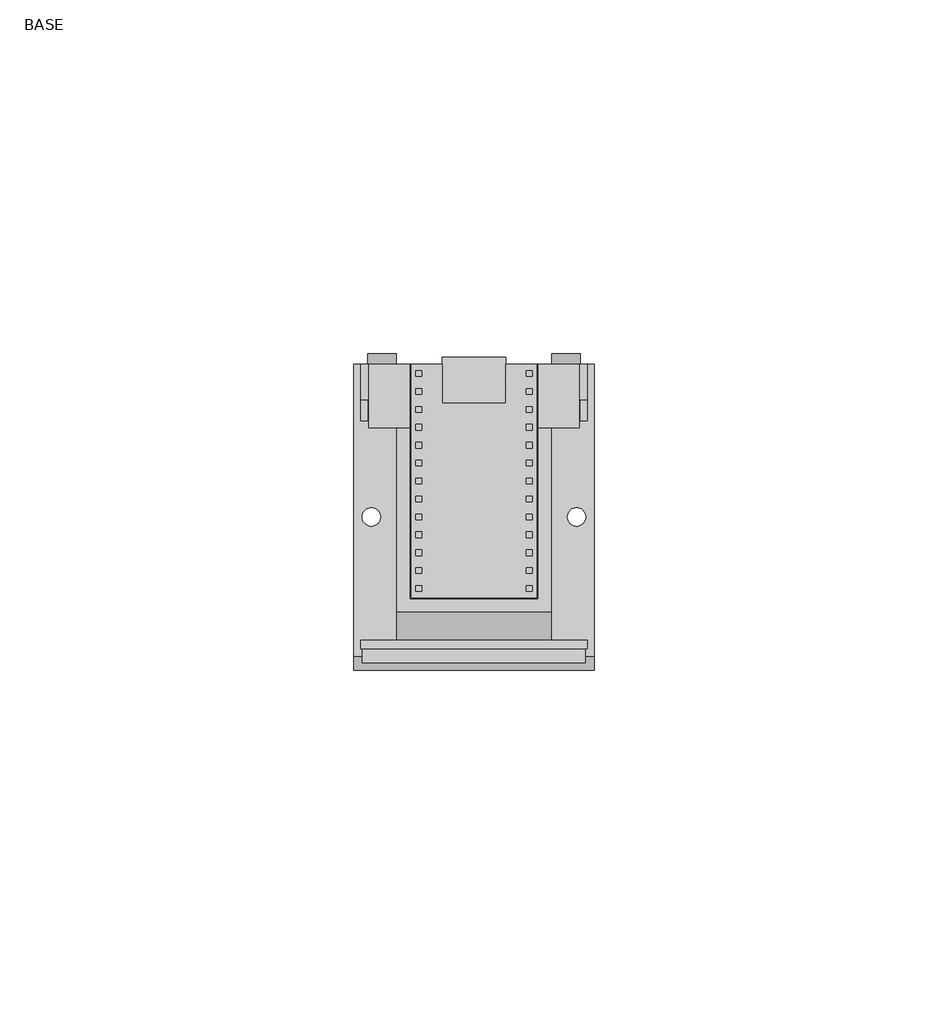
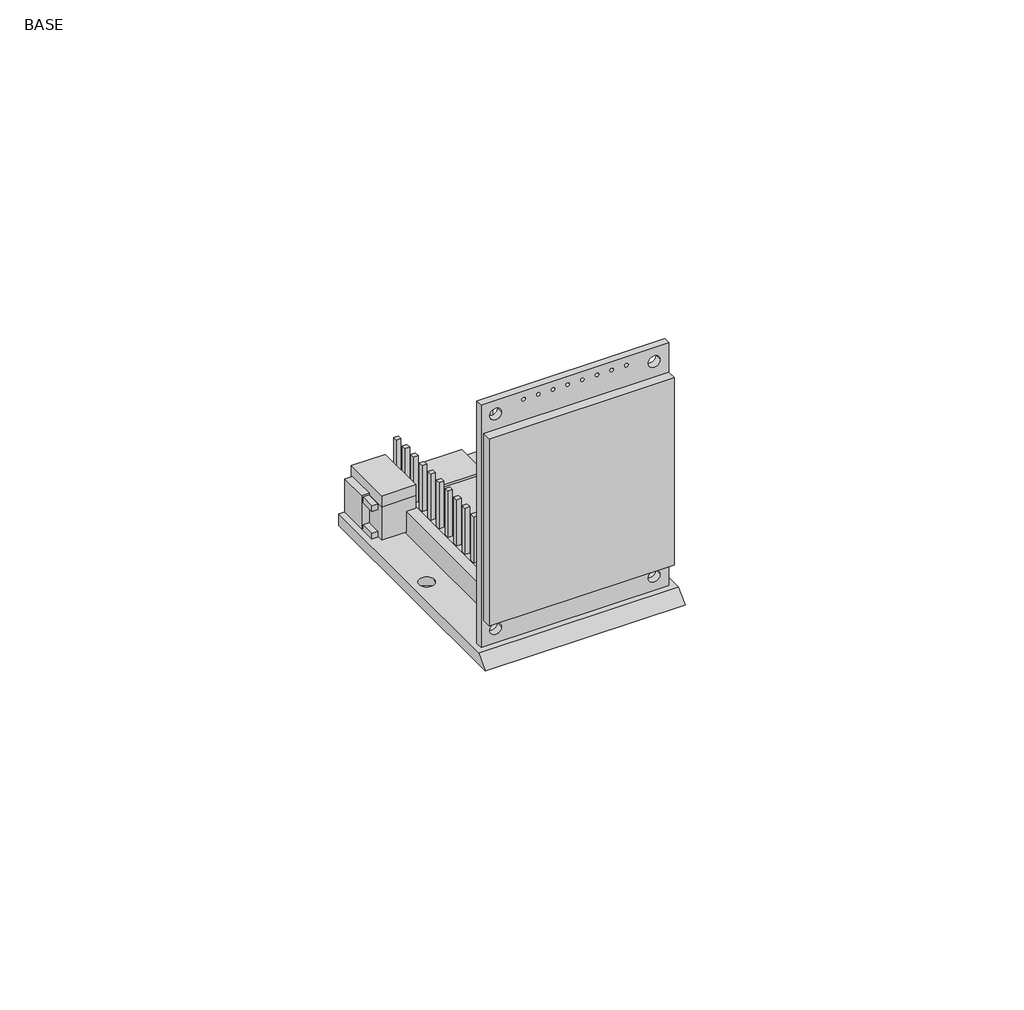
# One storey: 4 furniture elements, 1 proxy.
"""IFC4 building model written with IfcOpenShell, lengths in millimetres."""

import ifcopenshell
import ifcopenshell.guid

model = None  # the IFC model being written
_history = None  # IfcOwnerHistory: only IFC2X3 demands one
_inside = {}  # id of a spatial element -> (the spatial element, [elements in it])
_under = {}  # id of a project, library or spatial element -> (it, [spatial elements below it])
_declared = {}  # id of a project -> (the project, [libraries it declares])
_typed = {}  # id of a type object -> (the type object, [elements of that type])
_made_of = {}  # id of a material, layer set ... -> (it, [elements and type objects made of it])


def new_model(schema):
    """Start an empty IFC model of exactly this schema.

    Asked for "IFC4X3", IfcOpenShell would pick the latest addendum, in which some entities
    have other attributes; the version numbers below select the first issue.
    IFC2X3 requires an IfcOwnerHistory on every rooted entity: one is made here for all.
    """
    global model, _history
    if schema == "IFC4X3":
        model = ifcopenshell.file(schema_version=(4, 3, 0, 0))
    else:
        model = ifcopenshell.file(schema=schema)
    _inside.clear()
    _under.clear()
    _declared.clear()
    _typed.clear()
    _made_of.clear()
    _history = None
    if model.schema == "IFC2X3":
        org = make("IfcOrganization", Name="unknown")
        user = make(
            "IfcPersonAndOrganization",
            ThePerson=make("IfcPerson", FamilyName="unknown"),
            TheOrganization=org,
        )
        app = make(
            "IfcApplication",
            ApplicationDeveloper=org,
            Version="unknown",
            ApplicationFullName="unknown",
            ApplicationIdentifier="unknown",
        )
        _history = make(
            "IfcOwnerHistory",
            OwningUser=user,
            OwningApplication=app,
            ChangeAction="ADDED",
            CreationDate=0,
        )
    return model


def make(cls, **values):
    """One entity of the class cls with the attributes given. An attribute that is None is left unset."""
    return model.create_entity(
        cls, **{name: value for name, value in values.items() if value is not None}
    )


def rooted(cls, **values):
    """An entity with a GlobalId (a new one), such as an element, a storey or a relation."""
    return make(cls, GlobalId=ifcopenshell.guid.new(), OwnerHistory=_history, **values)


def si_unit(unit_type, name, prefix=None):
    """IfcSIUnit, for example si_unit("LENGTHUNIT", "METRE", prefix="MILLI")."""
    return make("IfcSIUnit", UnitType=unit_type, Prefix=prefix, Name=name)


def assignment(units):
    """IfcUnitAssignment: the units of a project."""
    return None if units is None else make("IfcUnitAssignment", Units=units)


def point(xyz):
    """IfcCartesianPoint."""
    return None if xyz is None else make("IfcCartesianPoint", Coordinates=xyz)


def direction(xyz):
    """IfcDirection."""
    return None if xyz is None else make("IfcDirection", DirectionRatios=xyz)


def frame(location, z_axis=None, x_axis=None):
    """IfcAxis2Placement3D, a coordinate frame: its origin and axes. An axis left out is left unset."""
    return make(
        "IfcAxis2Placement3D",
        Location=point(location),
        Axis=direction(z_axis),
        RefDirection=direction(x_axis),
    )


def frame_2d(location, x_axis=None):
    """IfcAxis2Placement2D, a coordinate frame in the plane: its origin and x axis."""
    return make(
        "IfcAxis2Placement2D", Location=point(location), RefDirection=direction(x_axis)
    )


def origin():
    """The frame at (0, 0, 0) with its axes left unset."""
    return frame((0.0, 0.0, 0.0))


def origin_with_axes():
    """The frame at (0, 0, 0) with the z axis (0, 0, 1) and the x axis (1, 0, 0) written out."""
    return frame((0.0, 0.0, 0.0), z_axis=(0.0, 0.0, 1.0), x_axis=(1.0, 0.0, 0.0))


def place(relative_to, where):
    """IfcLocalPlacement: puts the frame where relative to a parent placement (None: the world)."""
    return make(
        "IfcLocalPlacement", PlacementRelTo=relative_to, RelativePlacement=where
    )


def context(
    kind, dimensions, precision=None, world=None, true_north=None, identifier=None
):
    """IfcGeometricRepresentationContext, for example the 3D "Model" context."""
    return make(
        "IfcGeometricRepresentationContext",
        ContextIdentifier=identifier,
        ContextType=kind,
        CoordinateSpaceDimension=dimensions,
        Precision=precision,
        WorldCoordinateSystem=world,
        TrueNorth=true_north,
    )


def project(units=None, contexts=None):
    """IfcProject with its units and contexts."""
    return rooted(
        "IfcProject",
        Name="project",
        RepresentationContexts=contexts,
        UnitsInContext=assignment(units),
    )


def spatial(cls, under=None, at=None, **own):
    """A site, building, storey or space (cls), placed at a placement, below another one or the project."""
    s = rooted(cls, ObjectPlacement=at, **own)
    if under is not None:
        _under.setdefault(under.id(), (under, []))[1].append(s)
    return s


def polyline(points):
    """IfcPolyline through the points."""
    return make("IfcPolyline", Points=[point(p) for p in points])


def circle_curve(where, radius):
    """IfcCircle in the frame where."""
    return make("IfcCircle", Position=where, Radius=radius)


def trimmed(basis, trim1, trim2, sense, master):
    """IfcTrimmedCurve: the piece of a basis curve between two trims."""
    return make(
        "IfcTrimmedCurve",
        BasisCurve=basis,
        Trim1=trim1,
        Trim2=trim2,
        SenseAgreement=sense,
        MasterRepresentation=master,
    )


def segment(curve, same_sense, transition):
    """IfcCompositeCurveSegment."""
    return make(
        "IfcCompositeCurveSegment",
        Transition=transition,
        SameSense=same_sense,
        ParentCurve=curve,
    )


def composite_curve(segments, self_intersect=None):
    """IfcCompositeCurve: segments joined end to end."""
    return make("IfcCompositeCurve", Segments=segments, SelfIntersect=self_intersect)


def outline(outer, holes=None, kind="AREA"):
    """IfcArbitraryClosedProfileDef: a profile drawn as a closed curve; with holes, ...WithVoids."""
    if holes is None:
        return make("IfcArbitraryClosedProfileDef", ProfileType=kind, OuterCurve=outer)
    return make(
        "IfcArbitraryProfileDefWithVoids",
        ProfileType=kind,
        OuterCurve=outer,
        InnerCurves=holes,
    )


def extrude(swept, where, along, depth):
    """IfcExtrudedAreaSolid: the profile swept, set in the frame where, extruded along a direction by depth."""
    return make(
        "IfcExtrudedAreaSolid",
        SweptArea=swept,
        Position=where,
        ExtrudedDirection=direction(along),
        Depth=depth,
    )


def faces_of(points, faces, orient=None, outer=None):
    """IfcFace entities. A face is a list of loops; a loop is a list of indices into points, from 0.

    orient and outer hold one flag for each loop. By default every Orientation is true, the
    first loop of a face is its IfcFaceOuterBound and the others are IfcFaceBound.
    """
    made = []
    for i, loops in enumerate(faces):
        bounds = []
        for j, loop in enumerate(loops):
            is_outer = j == 0 if outer is None else outer[i][j]
            bounds.append(
                make(
                    "IfcFaceOuterBound" if is_outer else "IfcFaceBound",
                    Bound=make("IfcPolyLoop", Polygon=[points[k] for k in loop]),
                    Orientation=True if orient is None else orient[i][j],
                )
            )
        made.append(make("IfcFace", Bounds=bounds))
    return made


def faceted_brep(points, faces, orient=None, outer=None, voids=None):
    """IfcFacetedBrep: a solid bounded by flat faces; with voids (closed shells), ...WithVoids."""
    shared = [point(p) for p in points]
    hull = make("IfcClosedShell", CfsFaces=faces_of(shared, faces, orient, outer))
    if voids is None:
        return make("IfcFacetedBrep", Outer=hull)
    return make(
        "IfcFacetedBrepWithVoids",
        Outer=hull,
        Voids=[
            make(cls, CfsFaces=faces_of(shared, fs, o, b)) for cls, fs, o, b in voids
        ],
    )


def shape(context_of_items, identifier, shape_type, items):
    """IfcShapeRepresentation: the items that make up one representation, for example the "Body"."""
    return make(
        "IfcShapeRepresentation",
        ContextOfItems=context_of_items,
        RepresentationIdentifier=identifier,
        RepresentationType=shape_type,
        Items=items,
    )


def source(mapping_origin, context_of_items, identifier, shape_type, items):
    """IfcRepresentationMap: a shape defined once, which mapped items show again and again."""
    return make(
        "IfcRepresentationMap",
        MappingOrigin=mapping_origin,
        MappedRepresentation=shape(context_of_items, identifier, shape_type, items),
    )


def transform(
    local_origin,
    x_axis=None,
    y_axis=None,
    z_axis=None,
    scale=None,
    scale2=None,
    scale3=None,
    uniform=True,
):
    """IfcCartesianTransformationOperator3D, or its non-uniform kind. x_axis, y_axis, z_axis: its Axis1, 2, 3."""
    if uniform:
        return make(
            "IfcCartesianTransformationOperator3D",
            Axis1=direction(x_axis),
            Axis2=direction(y_axis),
            LocalOrigin=point(local_origin),
            Scale=scale,
            Axis3=direction(z_axis),
        )
    return make(
        "IfcCartesianTransformationOperator3DnonUniform",
        Axis1=direction(x_axis),
        Axis2=direction(y_axis),
        LocalOrigin=point(local_origin),
        Scale=scale,
        Axis3=direction(z_axis),
        Scale2=scale2,
        Scale3=scale3,
    )


def mapped(mapping_source, mapping_target):
    """IfcMappedItem: shows the shape of a source again, moved by a transform."""
    return make(
        "IfcMappedItem", MappingSource=mapping_source, MappingTarget=mapping_target
    )


def made_of(thing, what):
    """Note that an element or type object is made of a material, layer set ...; save() writes the relation."""
    if what is not None:
        _made_of.setdefault(what.id(), (what, []))[1].append(thing)
    return thing


def element(
    cls,
    number,
    at=None,
    inside=None,
    cuts=None,
    type_object=None,
    material=None,
    context=None,
    identifier="Body",
    shape_type=None,
    held_by="IfcProductDefinitionShape",
    body=None,
    shapes=None,
    **own,
):
    """One element of the class cls, such as IfcWall. Its Tag is "e" and its number.

    at: its placement. inside: the storey or other place that contains it. cuts: it is an
    opening in that element (IfcRelVoidsElement). A single representation is given by context,
    identifier, shape_type and body (its items); several are given by shapes. held_by: the class
    of the entity that holds the representations. save() writes the other relations.
    """
    e = rooted(cls, Tag="e%d" % number, ObjectPlacement=at, **own)
    if body is not None:
        shapes = [shape(context, identifier, shape_type, body)]
    if shapes is not None:
        e.Representation = make(held_by, Representations=shapes)
    if inside is not None:
        _inside.setdefault(inside.id(), (inside, []))[1].append(e)
    if cuts is not None:
        rooted(
            "IfcRelVoidsElement", RelatingBuildingElement=cuts, RelatedOpeningElement=e
        )
    if type_object is not None:
        _typed.setdefault(type_object.id(), (type_object, []))[1].append(e)
    return made_of(e, material)


def aggregate(whole, parts):
    """IfcRelAggregates: a whole, such as a stair, and the parts it consists of."""
    return rooted("IfcRelAggregates", RelatingObject=whole, RelatedObjects=parts)


def save(model, path):
    """Write the relations noted so far, then the file.

    IfcRelAggregates (storeys below a building ...), IfcRelContainedInSpatialStructure (elements
    in a storey), IfcRelDefinesByType, IfcRelAssociatesMaterial and IfcRelDeclares: one each for
    every whole, place, type object, material and project.
    """
    for whole, parts in _under.values():
        aggregate(whole, parts)
    for where, things in _inside.values():
        rooted(
            "IfcRelContainedInSpatialStructure",
            RelatedElements=things,
            RelatingStructure=where,
        )
    for kind, things in _typed.values():
        rooted("IfcRelDefinesByType", RelatedObjects=things, RelatingType=kind)
    for what, things in _made_of.values():
        rooted("IfcRelAssociatesMaterial", RelatedObjects=things, RelatingMaterial=what)
    for by, libraries in _declared.values():
        rooted("IfcRelDeclares", RelatingContext=by, RelatedDefinitions=libraries)
    model.write(path)


def plane_surface(at):
    """IfcPlane: the flat surface through the origin of the frame at, square to its z axis."""
    return make("IfcPlane", Position=at)


def revolved_surface(curve, axis_point, axis_direction):
    """IfcSurfaceOfRevolution: the curve turned about the line through axis_point along axis_direction."""
    return make(
        "IfcSurfaceOfRevolution",
        SweptCurve=make("IfcArbitraryOpenProfileDef", ProfileType="CURVE", Curve=curve),
        AxisPosition=make("IfcAxis1Placement", Location=point(axis_point), Axis=direction(axis_direction)),
    )


def advanced_brep(points, edges, surfaces, faces):
    """IfcAdvancedBrep: a solid bounded by faces that lie on surfaces and meet in shared edges.

    An edge is (start, end): straight between two places in points (the first is 0);
    or (start, end, curve); or (start, end, curve, False) where it runs against its curve.
    A face is (place in surfaces, loops), or (place, loops, False) where it looks against
    its surface's normal. A loop lists edges by number (the first is 1), with a minus sign
    where the edge is run from its end to its start. The first loop is the outer one.
    """
    corners = [point(p) for p in points]
    vertices = [make("IfcVertexPoint", VertexGeometry=c) for c in corners]
    made = []
    for start, end, *more in edges:
        made.append(
            make(
                "IfcEdgeCurve",
                EdgeStart=vertices[start],
                EdgeEnd=vertices[end],
                EdgeGeometry=more[0] if more else make("IfcPolyline", Points=[corners[start], corners[end]]),
                SameSense=more[1] if len(more) > 1 else True,
            )
        )
    hull = []
    for where, loops, *sense in faces:
        bounds = []
        for j, loop in enumerate(loops):
            ring = [make("IfcOrientedEdge", EdgeElement=made[abs(k) - 1], Orientation=k > 0) for k in loop]
            bounds.append(
                make(
                    "IfcFaceOuterBound" if j == 0 else "IfcFaceBound",
                    Bound=make("IfcEdgeLoop", EdgeList=ring),
                    Orientation=True,
                )
            )
        hull.append(make("IfcAdvancedFace", Bounds=bounds, FaceSurface=surfaces[where], SameSense=sense[0] if sense else True))
    return make("IfcAdvancedBrep", Outer=make("IfcClosedShell", CfsFaces=hull))


def case_case_fa127987(model_context):
    return source(origin(), model_context, "Body", "SolidModel", [
        extrude(outline(polyline([(1442.9350176, 13234.6739696), (1442.9350176, 13225.7186096), (1437.1350176, 13225.7186096), (1437.1350176, 13234.6739696), (1442.9350176, 13234.6739696)])), frame((0.0, 0.0, 8.0), z_axis=(0.0, 0.0, 1.0), x_axis=(1.0, 0.0, 0.0)), (0.0, 0.0, 1.0), 2.0),
        extrude(outline(polyline([(1461.1150176, 13234.6739696), (1466.9150176, 13234.6739696), (1466.9150176, 13225.7186096), (1461.1150176, 13225.7186096), (1461.1150176, 13234.6739696)])), frame((0.0, 0.0, 8.0), z_axis=(0.0, 0.0, 1.0), x_axis=(1.0, 0.0, 0.0)), (0.0, 0.0, 1.0), 2.0),
        extrude(outline(polyline([(1442.9350176, 13230.2186096), (1442.9350176, 13225.7186096), (1437.1350176, 13225.7186096), (1437.1350176, 13230.2186096), (1442.9350176, 13230.2186096)])), frame((0.0, 0.0, 2.0), z_axis=(0.0, 0.0, 1.0), x_axis=(1.0, 0.0, 0.0)), (0.0, 0.0, 1.0), 6.0),
        extrude(outline(polyline([(1461.1150176, 13230.2186096), (1466.9150176, 13230.2186096), (1466.9150176, 13225.7186096), (1461.1150176, 13225.7186096), (1461.1150176, 13230.2186096)])), frame((0.0, 0.0, 2.0), z_axis=(0.0, 0.0, 1.0), x_axis=(1.0, 0.0, 0.0)), (0.0, 0.0, 1.0), 6.0),
        advanced_brep(
        [(1469.0250176, 13193.4256546, 2.0), (1469.0250176, 13234.6739696, 2.0), (1435.0250176, 13234.6739696, 2.0), (1435.0250176, 13193.4256546, 2.0), (1441.1350176, 13195.6739696, 2.0), (1441.1350176, 13225.7186096, 2.0), (1442.9350176, 13225.7186096, 2.0), (1442.9350176, 13201.4739696, 2.0), (1461.1150176, 13201.4739696, 2.0), (1461.1150176, 13225.7186096, 2.0), (1462.9150176, 13225.7186096, 2.0), (1462.9150176, 13195.6739696, 2.0), (1467.8250176, 13213.1041412, 2.0), (1465.2250176, 13213.1041412, 2.0), (1438.8250176, 13213.1041412, 2.0), (1436.2250176, 13213.1041412, 2.0), (1435.0250176, 13234.6739696, 0.0), (1469.0250176, 13234.6739696, 0.0), (1469.0250176, 13191.4256546, 0.0), (1435.0250176, 13191.4256546, 0.0), (1464.5250176, 13213.1041412, 0.0), (1468.5250176, 13213.1041412, 0.0), (1435.5250176, 13213.1041412, 0.0), (1439.5250176, 13213.1041412, 0.0), (1441.1350176, 13225.7186096, 6.0), (1441.1350176, 13199.6739696, 6.0), (1462.9150176, 13199.6739696, 6.0), (1462.9150176, 13225.7186096, 6.0), (1461.1150176, 13225.7186096, 6.0), (1461.1150176, 13201.4739696, 6.0), (1442.9350176, 13201.4739696, 6.0), (1442.9350176, 13225.7186096, 6.0)],
        [
            (0, 1),
            (1, 2),
            (2, 3),
            (3, 0),
            (4, 5),
            (5, 6),
            (6, 7),
            (7, 8),
            (8, 9),
            (9, 10),
            (10, 11),
            (11, 4),
            (12, 13, circle_curve(frame((1466.5250176, 13213.1041412, 2.0), z_axis=(0.0, 0.0, -1.0), x_axis=(-1.0, 0.0, 0.0)), 1.3)),
            (13, 12, circle_curve(frame((1466.5250176, 13213.1041412, 2.0), z_axis=(0.0, 0.0, -1.0), x_axis=(1.0, 0.0, 0.0)), 1.3)),
            (14, 15, circle_curve(frame((1437.5250176, 13213.1041412, 2.0), z_axis=(0.0, 0.0, -1.0), x_axis=(-1.0, 0.0, 0.0)), 1.3)),
            (15, 14, circle_curve(frame((1437.5250176, 13213.1041412, 2.0), z_axis=(0.0, 0.0, -1.0), x_axis=(1.0, 0.0, 0.0)), 1.3)),
            (16, 17),
            (17, 18),
            (18, 19),
            (19, 16),
            (20, 21, circle_curve(frame((1466.5250176, 13213.1041412, 0.0), z_axis=(0.0, 0.0, 1.0), x_axis=(-1.0, 0.0, 0.0)), 2.0)),
            (21, 20, circle_curve(frame((1466.5250176, 13213.1041412, 0.0), z_axis=(0.0, 0.0, 1.0), x_axis=(1.0, 0.0, 0.0)), 2.0)),
            (22, 23, circle_curve(frame((1437.5250176, 13213.1041412, 0.0), z_axis=(0.0, 0.0, 1.0), x_axis=(-1.0, 0.0, 0.0)), 2.0)),
            (23, 22, circle_curve(frame((1437.5250176, 13213.1041412, 0.0), z_axis=(0.0, 0.0, 1.0), x_axis=(1.0, 0.0, 0.0)), 2.0)),
            (0, 18),
            (17, 1),
            (16, 2),
            (19, 3),
            (24, 25),
            (25, 26),
            (26, 27),
            (27, 28),
            (28, 29),
            (29, 30),
            (30, 31),
            (31, 24),
            (24, 5),
            (4, 25),
            (26, 11),
            (10, 27),
            (9, 28),
            (8, 29),
            (7, 30),
            (6, 31),
            (20, 13),
            (12, 21),
            (22, 15),
            (14, 23),
        ],
        [
            plane_surface(frame((1467.7850176, 13193.4256546, 2.0), z_axis=(0.0, 0.0, 1.0), x_axis=(1.0, 0.0, 0.0))),
            plane_surface(frame((1467.7850176, 13193.4256546, 0.0), z_axis=(0.0, 0.0, -1.0), x_axis=(-1.0, 0.0, 0.0))),
            plane_surface(frame((1469.0250176, 13193.4256546, 2.0), z_axis=(1.0, 0.0, 0.0), x_axis=(0.0, 0.0, -1.0))),
            plane_surface(frame((1469.0250176, 13234.6739696, 2.0), z_axis=(0.0, 1.0, 0.0), x_axis=(0.0, 0.0, -1.0))),
            plane_surface(frame((1435.0250176, 13234.6739696, 2.0), z_axis=(-1.0, 0.0, 0.0), x_axis=(0.0, 0.0, -1.0))),
            plane_surface(frame((1441.1350176, 13234.6739696, 6.0), z_axis=(0.0, 0.0, 1.0), x_axis=(0.0, -1.0, 0.0))),
            plane_surface(frame((1441.1350176, 13225.7186096, 6.0), z_axis=(-1.0, 0.0, 0.0), x_axis=(0.0, 0.0, -1.0))),
            plane_surface(frame((1462.9150176, 13199.6739696, 6.0), z_axis=(1.0, 0.0, 0.0), x_axis=(0.0, 0.0, -1.0))),
            plane_surface(frame((1462.9150176, 13225.7186096, 6.0), z_axis=(0.0, 1.0, 0.0), x_axis=(0.0, 0.0, -1.0))),
            plane_surface(frame((1461.1150176, 13225.7186096, 6.0), z_axis=(-1.0, 0.0, 0.0), x_axis=(0.0, 0.0, -1.0))),
            plane_surface(frame((1461.1150176, 13201.4739696, 6.0), z_axis=(0.0, 1.0, 0.0), x_axis=(0.0, 0.0, -1.0))),
            plane_surface(frame((1442.9350176, 13201.4739696, 6.0), z_axis=(1.0, 0.0, 0.0), x_axis=(0.0, 0.0, -1.0))),
            plane_surface(frame((1442.9350176, 13225.7186096, 6.0), z_axis=(0.0, 1.0, 0.0), x_axis=(0.0, 0.0, -1.0))),
            plane_surface(frame((1441.1350176, 13195.6739696, 2.0), z_axis=(0.0, -0.7071067811865885, 0.7071067811865066), x_axis=(1.0, 0.0, 0.0))),
            revolved_surface(polyline([(1464.5250176, 13213.1041412, 0.0), (1465.2250176017499, 13213.1041412, 2.0)]), (1466.5250176, 13213.1041412, 5.7142857), (0.0, 0.0, -1.0)),
            revolved_surface(polyline([(1435.5250176, 13213.1041412, 0.0), (1436.2250176017499, 13213.1041412, 2.0)]), (1437.5250176, 13213.1041412, 5.7142857), (0.0, 0.0, -1.0)),
            plane_surface(frame((1435.0250176, 13191.4256546, 0.0), z_axis=(0.0, -0.707106781186628, 0.7071067811864672), x_axis=(1.0, 0.0, 0.0))),
        ],
        [
            (0, [[1, 2, 3, 4], [5, 6, 7, 8, 9, 10, 11, 12], [13, 14], [15, 16]]),
            (1, [[17, 18, 19, 20], [21, 22], [23, 24]]),
            (2, [[-1, 25, -18, 26]]),
            (3, [[-2, -26, -17, 27]]),
            (4, [[-3, -27, -20, 28]]),
            (5, [[29, 30, 31, 32, 33, 34, 35, 36]]),
            (6, [[-29, 37, -5, 38]]),
            (7, [[-31, 39, -11, 40]]),
            (8, [[-32, -40, -10, 41]]),
            (9, [[-33, -41, -9, 42]]),
            (10, [[-34, -42, -8, 43]]),
            (11, [[-35, -43, -7, 44]]),
            (12, [[-36, -44, -6, -37]]),
            (13, [[-38, -12, -39, -30]]),
            (14, [[45, -13, 46, -21]]),
            (14, [[-45, -22, -46, -14]]),
            (15, [[47, -15, 48, -23]]),
            (15, [[-47, -24, -48, -16]]),
            (16, [[-28, -19, -25, -4]]),
        ],
    ),
    ])


def furniture_1_54tft_screen_1_54tft_screen_d9e98271(model_context):
    return source(origin(), model_context, "Body", "SweptSolid", [
        extrude(outline(polyline([(43.7, 16.0), (43.7, -16.0), (0.0, -16.0), (0.0, 16.0), (43.7, 16.0)]), holes=[composite_curve([segment(trimmed(circle_curve(frame_2d((2.5, 13.5)), 1.0), [point((2.5, 14.5))], [point((2.5, 12.5))], True, "CARTESIAN"), True, "CONTINUOUS"), segment(trimmed(circle_curve(frame_2d((2.5, 13.5)), 1.0), [point((2.5, 12.5))], [point((2.5, 14.5))], True, "CARTESIAN"), True, "CONTINUOUS")], self_intersect=False), composite_curve([segment(trimmed(circle_curve(frame_2d((41.2, 13.5)), 1.0), [point((41.2, 14.5))], [point((41.2, 12.5))], True, "CARTESIAN"), True, "CONTINUOUS"), segment(trimmed(circle_curve(frame_2d((41.2, 13.5)), 1.0), [point((41.2, 12.5))], [point((41.2, 14.5))], True, "CARTESIAN"), True, "CONTINUOUS")], self_intersect=False), composite_curve([segment(trimmed(circle_curve(frame_2d((42.2, -1.25)), 0.3), [point((42.2, -0.95))], [point((42.2, -1.55))], True, "CARTESIAN"), True, "CONTINUOUS"), segment(trimmed(circle_curve(frame_2d((42.2, -1.25)), 0.3), [point((42.2, -1.55))], [point((42.2, -0.95))], True, "CARTESIAN"), True, "CONTINUOUS")], self_intersect=False), composite_curve([segment(trimmed(circle_curve(frame_2d((42.2, 1.25)), 0.3), [point((42.2, 1.55))], [point((42.2, 0.95))], True, "CARTESIAN"), True, "CONTINUOUS"), segment(trimmed(circle_curve(frame_2d((42.2, 1.25)), 0.3), [point((42.2, 0.95))], [point((42.2, 1.55))], True, "CARTESIAN"), True, "CONTINUOUS")], self_intersect=False), composite_curve([segment(trimmed(circle_curve(frame_2d((42.2, 3.75)), 0.3), [point((42.2, 4.05))], [point((42.2, 3.45))], True, "CARTESIAN"), True, "CONTINUOUS"), segment(trimmed(circle_curve(frame_2d((42.2, 3.75)), 0.3), [point((42.2, 3.45))], [point((42.2, 4.05))], True, "CARTESIAN"), True, "CONTINUOUS")], self_intersect=False), composite_curve([segment(trimmed(circle_curve(frame_2d((42.2, 6.25)), 0.3), [point((42.2, 6.55))], [point((42.2, 5.95))], True, "CARTESIAN"), True, "CONTINUOUS"), segment(trimmed(circle_curve(frame_2d((42.2, 6.25)), 0.3), [point((42.2, 5.95))], [point((42.2, 6.55))], True, "CARTESIAN"), True, "CONTINUOUS")], self_intersect=False), composite_curve([segment(trimmed(circle_curve(frame_2d((42.2, 8.75)), 0.3), [point((42.2, 9.05))], [point((42.2, 8.45))], True, "CARTESIAN"), True, "CONTINUOUS"), segment(trimmed(circle_curve(frame_2d((42.2, 8.75)), 0.3), [point((42.2, 8.45))], [point((42.2, 9.05))], True, "CARTESIAN"), True, "CONTINUOUS")], self_intersect=False), composite_curve([segment(trimmed(circle_curve(frame_2d((42.2, -3.75)), 0.3), [point((42.2, -3.45))], [point((42.2, -4.05))], True, "CARTESIAN"), True, "CONTINUOUS"), segment(trimmed(circle_curve(frame_2d((42.2, -3.75)), 0.3), [point((42.2, -4.05))], [point((42.2, -3.45))], True, "CARTESIAN"), True, "CONTINUOUS")], self_intersect=False), composite_curve([segment(trimmed(circle_curve(frame_2d((42.2, -6.25)), 0.3), [point((42.2, -5.95))], [point((42.2, -6.55))], True, "CARTESIAN"), True, "CONTINUOUS"), segment(trimmed(circle_curve(frame_2d((42.2, -6.25)), 0.3), [point((42.2, -6.55))], [point((42.2, -5.95))], True, "CARTESIAN"), True, "CONTINUOUS")], self_intersect=False), composite_curve([segment(trimmed(circle_curve(frame_2d((42.2, -8.75)), 0.3), [point((42.2, -8.45))], [point((42.2, -9.05))], True, "CARTESIAN"), True, "CONTINUOUS"), segment(trimmed(circle_curve(frame_2d((42.2, -8.75)), 0.3), [point((42.2, -9.05))], [point((42.2, -8.45))], True, "CARTESIAN"), True, "CONTINUOUS")], self_intersect=False), composite_curve([segment(trimmed(circle_curve(frame_2d((41.2, -13.5)), 1.0), [point((41.2, -14.5))], [point((41.2, -12.5))], True, "CARTESIAN"), True, "CONTINUOUS"), segment(trimmed(circle_curve(frame_2d((41.2, -13.5)), 1.0), [point((41.2, -12.5))], [point((41.2, -14.5))], True, "CARTESIAN"), True, "CONTINUOUS")], self_intersect=False), composite_curve([segment(trimmed(circle_curve(frame_2d((2.5, -13.5)), 1.0), [point((2.5, -14.5))], [point((2.5, -12.5))], True, "CARTESIAN"), True, "CONTINUOUS"), segment(trimmed(circle_curve(frame_2d((2.5, -13.5)), 1.0), [point((2.5, -12.5))], [point((2.5, -14.5))], True, "CARTESIAN"), True, "CONTINUOUS")], self_intersect=False)]), frame((0.0, -1.2, 0.0), z_axis=(0.0, 1.0, 0.0), x_axis=(0.0, 0.0, 1.0)), (0.0, 0.0, 1.0), 1.2),
        extrude(outline(polyline([(15.76, -1.3), (15.76, -3.2), (-15.76, -3.2), (-15.76, -1.3), (15.76, -1.3)])), frame((0.0, 0.0, 5.0), z_axis=(0.0, 0.0, 1.0), x_axis=(1.0, 0.0, 0.0)), (0.0, 0.0, 1.0), 33.7),
        extrude(outline(polyline([(13.86, -2.3592442), (13.86, -3.2), (-13.86, -3.2), (-13.86, -2.3592442), (13.86, -2.3592442)])), frame((0.0, 0.0, 9.5994076), z_axis=(0.0, 0.0, 1.0), x_axis=(1.0, 0.0, 0.0)), (0.0, 0.0, 1.0), 27.7),
    ])


def pro_micro_nrf52840_pro_micro_nrf52840_bcfd0b97(model_context):
    return source(origin(), model_context, "Body", "Brep", [
        faceted_brep([(-14.8, 8.2144911, 11.3), (-15.6, 8.2144911, 11.3), (-15.6, 7.4144911, 11.3), (-14.8, 7.4144911, 11.3), (15.6, 8.2144911, 11.3), (14.8, 8.2144911, 11.3), (14.8, 7.4144911, 11.3), (15.6, 7.4144911, 11.3), (13.0666667, 8.2144911, 11.3), (12.2666667, 8.2144911, 11.3), (12.2666667, 7.4144911, 11.3), (13.0666667, 7.4144911, 11.3), (10.5333333, 8.2144911, 11.3), (9.7333333, 8.2144911, 11.3), (9.7333333, 7.4144911, 11.3), (10.5333333, 7.4144911, 11.3), (8.0, 8.2144911, 11.3), (7.2, 8.2144911, 11.3), (7.2, 7.4144911, 11.3), (8.0, 7.4144911, 11.3), (5.4666667, 8.2144911, 11.3), (4.6666667, 8.2144911, 11.3), (4.6666667, 7.4144911, 11.3), (5.4666667, 7.4144911, 11.3), (2.9333333, 8.2144911, 11.3), (2.1333333, 8.2144911, 11.3), (2.1333333, 7.4144911, 11.3), (2.9333333, 7.4144911, 11.3), (0.4, 8.2144911, 11.3), (-0.4, 8.2144911, 11.3), (-0.4, 7.4144911, 11.3), (0.4, 7.4144911, 11.3), (-2.1333333, 8.2144911, 11.3), (-2.9333333, 8.2144911, 11.3), (-2.9333333, 7.4144911, 11.3), (-2.1333333, 7.4144911, 11.3), (-4.6666667, 8.2144911, 11.3), (-5.4666667, 8.2144911, 11.3), (-5.4666667, 7.4144911, 11.3), (-4.6666667, 7.4144911, 11.3), (-7.2, 8.2144911, 11.3), (-8.0, 8.2144911, 11.3), (-8.0, 7.4144911, 11.3), (-7.2, 7.4144911, 11.3), (-9.7333333, 8.2144911, 11.3), (-10.5333333, 8.2144911, 11.3), (-10.5333333, 7.4144911, 11.3), (-9.7333333, 7.4144911, 11.3), (-12.2666667, 8.2144911, 11.3), (-13.0666667, 8.2144911, 11.3), (-13.0666667, 7.4144911, 11.3), (-12.2666667, 7.4144911, 11.3), (-14.8, 8.2144911, 0.0), (-14.8, 7.4144911, 0.0), (-15.6, 7.4144911, 0.0), (-15.6, 8.2144911, 0.0), (15.6, 8.2144911, 0.0), (15.6, 7.4144911, 0.0), (14.8, 7.4144911, 0.0), (14.8, 8.2144911, 0.0), (13.0666667, 8.2144911, 0.0), (13.0666667, 7.4144911, 0.0), (12.2666667, 7.4144911, 0.0), (12.2666667, 8.2144911, 0.0), (10.5333333, 8.2144911, 0.0), (10.5333333, 7.4144911, 0.0), (9.7333333, 7.4144911, 0.0), (9.7333333, 8.2144911, 0.0), (8.0, 8.2144911, 0.0), (8.0, 7.4144911, 0.0), (7.2, 7.4144911, 0.0), (7.2, 8.2144911, 0.0), (5.4666667, 8.2144911, 0.0), (5.4666667, 7.4144911, 0.0), (4.6666667, 7.4144911, 0.0), (4.6666667, 8.2144911, 0.0), (2.9333333, 8.2144911, 0.0), (2.9333333, 7.4144911, 0.0), (2.1333333, 7.4144911, 0.0), (2.1333333, 8.2144911, 0.0), (0.4, 8.2144911, 0.0), (0.4, 7.4144911, 0.0), (-0.4, 7.4144911, 0.0), (-0.4, 8.2144911, 0.0), (-2.1333333, 8.2144911, 0.0), (-2.1333333, 7.4144911, 0.0), (-2.9333333, 7.4144911, 0.0), (-2.9333333, 8.2144911, 0.0), (-4.6666667, 8.2144911, 0.0), (-4.6666667, 7.4144911, 0.0), (-5.4666667, 7.4144911, 0.0), (-5.4666667, 8.2144911, 0.0), (-7.2, 8.2144911, 0.0), (-7.2, 7.4144911, 0.0), (-8.0, 7.4144911, 0.0), (-8.0, 8.2144911, 0.0), (-9.7333333, 8.2144911, 0.0), (-9.7333333, 7.4144911, 0.0), (-10.5333333, 7.4144911, 0.0), (-10.5333333, 8.2144911, 0.0), (-12.2666667, 8.2144911, 0.0), (-12.2666667, 7.4144911, 0.0), (-13.0666667, 7.4144911, 0.0), (-13.0666667, 8.2144911, 0.0), (-14.8, 8.2144911, 3.0), (-15.6, 8.2144911, 3.0), (-15.6, 8.2144911, 1.0), (-14.8, 8.2144911, 1.0), (-15.6, 7.4144911, 3.0), (-15.6, 7.4144911, 1.0), (-14.8, 7.4144911, 3.0), (-14.8, 7.4144911, 1.0), (15.6, 8.2144911, 3.0), (14.8, 8.2144911, 3.0), (14.8, 8.2144911, 1.0), (15.6, 8.2144911, 1.0), (14.8, 7.4144911, 3.0), (14.8, 7.4144911, 1.0), (15.6, 7.4144911, 3.0), (15.6, 7.4144911, 1.0), (13.0666667, 8.2144911, 3.0), (12.2666667, 8.2144911, 3.0), (12.2666667, 8.2144911, 1.0), (13.0666667, 8.2144911, 1.0), (12.2666667, 7.4144911, 3.0), (12.2666667, 7.4144911, 1.0), (13.0666667, 7.4144911, 3.0), (13.0666667, 7.4144911, 1.0), (10.5333333, 8.2144911, 3.0), (9.7333333, 8.2144911, 3.0), (9.7333333, 8.2144911, 1.0), (10.5333333, 8.2144911, 1.0), (9.7333333, 7.4144911, 3.0), (9.7333333, 7.4144911, 1.0), (10.5333333, 7.4144911, 3.0), (10.5333333, 7.4144911, 1.0), (8.0, 8.2144911, 3.0), (7.2, 8.2144911, 3.0), (7.2, 8.2144911, 1.0), (8.0, 8.2144911, 1.0), (7.2, 7.4144911, 3.0), (7.2, 7.4144911, 1.0), (8.0, 7.4144911, 3.0), (8.0, 7.4144911, 1.0), (5.4666667, 8.2144911, 3.0), (4.6666667, 8.2144911, 3.0), (4.6666667, 8.2144911, 1.0), (5.4666667, 8.2144911, 1.0), (4.6666667, 7.4144911, 3.0), (4.6666667, 7.4144911, 1.0), (5.4666667, 7.4144911, 3.0), (5.4666667, 7.4144911, 1.0), (2.9333333, 8.2144911, 3.0), (2.1333333, 8.2144911, 3.0), (2.1333333, 8.2144911, 1.0), (2.9333333, 8.2144911, 1.0), (2.1333333, 7.4144911, 3.0), (2.1333333, 7.4144911, 1.0), (2.9333333, 7.4144911, 3.0), (2.9333333, 7.4144911, 1.0), (0.4, 8.2144911, 3.0), (-0.4, 8.2144911, 3.0), (-0.4, 8.2144911, 1.0), (0.4, 8.2144911, 1.0), (-0.4, 7.4144911, 3.0), (-0.4, 7.4144911, 1.0), (0.4, 7.4144911, 3.0), (0.4, 7.4144911, 1.0), (-2.1333333, 8.2144911, 3.0), (-2.9333333, 8.2144911, 3.0), (-2.9333333, 8.2144911, 1.0), (-2.1333333, 8.2144911, 1.0), (-2.9333333, 7.4144911, 3.0), (-2.9333333, 7.4144911, 1.0), (-2.1333333, 7.4144911, 3.0), (-2.1333333, 7.4144911, 1.0), (-4.6666667, 8.2144911, 3.0), (-5.4666667, 8.2144911, 3.0), (-5.4666667, 8.2144911, 1.0), (-4.6666667, 8.2144911, 1.0), (-5.4666667, 7.4144911, 3.0), (-5.4666667, 7.4144911, 1.0), (-4.6666667, 7.4144911, 3.0), (-4.6666667, 7.4144911, 1.0), (-7.2, 8.2144911, 3.0), (-8.0, 8.2144911, 3.0), (-8.0, 8.2144911, 1.0), (-7.2, 8.2144911, 1.0), (-8.0, 7.4144911, 3.0), (-8.0, 7.4144911, 1.0), (-7.2, 7.4144911, 3.0), (-7.2, 7.4144911, 1.0), (-9.7333333, 8.2144911, 3.0), (-10.5333333, 8.2144911, 3.0), (-10.5333333, 8.2144911, 1.0), (-9.7333333, 8.2144911, 1.0), (-10.5333333, 7.4144911, 3.0), (-10.5333333, 7.4144911, 1.0), (-9.7333333, 7.4144911, 3.0), (-9.7333333, 7.4144911, 1.0), (-12.2666667, 8.2144911, 3.0), (-13.0666667, 8.2144911, 3.0), (-13.0666667, 8.2144911, 1.0), (-12.2666667, 8.2144911, 1.0), (-13.0666667, 7.4144911, 3.0), (-13.0666667, 7.4144911, 1.0), (-12.2666667, 7.4144911, 3.0), (-12.2666667, 7.4144911, 1.0), (16.5, 8.89, 3.0), (-16.5, 8.89, 3.0), (-16.5, -8.89, 3.0), (16.5, -8.89, 3.0), (16.5, -4.5, 3.0), (11.0, -4.5, 3.0), (11.0, 4.5, 3.0), (16.5, 4.5, 3.0), (-14.8, -8.2144911, 3.0), (-15.6, -8.2144911, 3.0), (-15.6, -7.4144911, 3.0), (-14.8, -7.4144911, 3.0), (15.6, -8.2144911, 3.0), (14.8, -8.2144911, 3.0), (14.8, -7.4144911, 3.0), (15.6, -7.4144911, 3.0), (13.0666667, -8.2144911, 3.0), (12.2666667, -8.2144911, 3.0), (12.2666667, -7.4144911, 3.0), (13.0666667, -7.4144911, 3.0), (10.5333333, -8.2144911, 3.0), (9.7333333, -8.2144911, 3.0), (9.7333333, -7.4144911, 3.0), (10.5333333, -7.4144911, 3.0), (8.0, -8.2144911, 3.0), (7.2, -8.2144911, 3.0), (7.2, -7.4144911, 3.0), (8.0, -7.4144911, 3.0), (5.4666667, -8.2144911, 3.0), (4.6666667, -8.2144911, 3.0), (4.6666667, -7.4144911, 3.0), (5.4666667, -7.4144911, 3.0), (2.9333333, -8.2144911, 3.0), (2.1333333, -8.2144911, 3.0), (2.1333333, -7.4144911, 3.0), (2.9333333, -7.4144911, 3.0), (0.4, -8.2144911, 3.0), (-0.4, -8.2144911, 3.0), (-0.4, -7.4144911, 3.0), (0.4, -7.4144911, 3.0), (-2.1333333, -8.2144911, 3.0), (-2.9333333, -8.2144911, 3.0), (-2.9333333, -7.4144911, 3.0), (-2.1333333, -7.4144911, 3.0), (-4.6666667, -8.2144911, 3.0), (-5.4666667, -8.2144911, 3.0), (-5.4666667, -7.4144911, 3.0), (-4.6666667, -7.4144911, 3.0), (-7.2, -8.2144911, 3.0), (-8.0, -8.2144911, 3.0), (-8.0, -7.4144911, 3.0), (-7.2, -7.4144911, 3.0), (-9.7333333, -8.2144911, 3.0), (-10.5333333, -8.2144911, 3.0), (-10.5333333, -7.4144911, 3.0), (-9.7333333, -7.4144911, 3.0), (-12.2666667, -8.2144911, 3.0), (-13.0666667, -8.2144911, 3.0), (-13.0666667, -7.4144911, 3.0), (-12.2666667, -7.4144911, 3.0), (16.5, -8.89, 1.0), (-16.5, -8.89, 1.0), (-16.5, 8.89, 1.0), (16.5, 8.89, 1.0), (16.5, 4.5, 1.0), (11.0, 4.5, 1.0), (11.0, -4.5, 1.0), (16.5, -4.5, 1.0), (-15.6, -8.2144911, 1.0), (-14.8, -8.2144911, 1.0), (-14.8, -7.4144911, 1.0), (-15.6, -7.4144911, 1.0), (14.8, -8.2144911, 1.0), (15.6, -8.2144911, 1.0), (15.6, -7.4144911, 1.0), (14.8, -7.4144911, 1.0), (12.2666667, -8.2144911, 1.0), (13.0666667, -8.2144911, 1.0), (13.0666667, -7.4144911, 1.0), (12.2666667, -7.4144911, 1.0), (9.7333333, -8.2144911, 1.0), (10.5333333, -8.2144911, 1.0), (10.5333333, -7.4144911, 1.0), (9.7333333, -7.4144911, 1.0), (7.2, -8.2144911, 1.0), (8.0, -8.2144911, 1.0), (8.0, -7.4144911, 1.0), (7.2, -7.4144911, 1.0), (4.6666667, -8.2144911, 1.0), (5.4666667, -8.2144911, 1.0), (5.4666667, -7.4144911, 1.0), (4.6666667, -7.4144911, 1.0), (2.1333333, -8.2144911, 1.0), (2.9333333, -8.2144911, 1.0), (2.9333333, -7.4144911, 1.0), (2.1333333, -7.4144911, 1.0), (-0.4, -8.2144911, 1.0), (0.4, -8.2144911, 1.0), (0.4, -7.4144911, 1.0), (-0.4, -7.4144911, 1.0), (-2.9333333, -8.2144911, 1.0), (-2.1333333, -8.2144911, 1.0), (-2.1333333, -7.4144911, 1.0), (-2.9333333, -7.4144911, 1.0), (-5.4666667, -8.2144911, 1.0), (-4.6666667, -8.2144911, 1.0), (-4.6666667, -7.4144911, 1.0), (-5.4666667, -7.4144911, 1.0), (-8.0, -8.2144911, 1.0), (-7.2, -8.2144911, 1.0), (-7.2, -7.4144911, 1.0), (-8.0, -7.4144911, 1.0), (-10.5333333, -8.2144911, 1.0), (-9.7333333, -8.2144911, 1.0), (-9.7333333, -7.4144911, 1.0), (-10.5333333, -7.4144911, 1.0), (-13.0666667, -8.2144911, 1.0), (-12.2666667, -8.2144911, 1.0), (-12.2666667, -7.4144911, 1.0), (-13.0666667, -7.4144911, 1.0), (-14.8, -8.2144911, 11.3), (-14.8, -7.4144911, 11.3), (-15.6, -7.4144911, 11.3), (-15.6, -8.2144911, 11.3), (15.6, -8.2144911, 11.3), (15.6, -7.4144911, 11.3), (14.8, -7.4144911, 11.3), (14.8, -8.2144911, 11.3), (13.0666667, -8.2144911, 11.3), (13.0666667, -7.4144911, 11.3), (12.2666667, -7.4144911, 11.3), (12.2666667, -8.2144911, 11.3), (10.5333333, -8.2144911, 11.3), (10.5333333, -7.4144911, 11.3), (9.7333333, -7.4144911, 11.3), (9.7333333, -8.2144911, 11.3), (8.0, -8.2144911, 11.3), (8.0, -7.4144911, 11.3), (7.2, -7.4144911, 11.3), (7.2, -8.2144911, 11.3), (5.4666667, -8.2144911, 11.3), (5.4666667, -7.4144911, 11.3), (4.6666667, -7.4144911, 11.3), (4.6666667, -8.2144911, 11.3), (2.9333333, -8.2144911, 11.3), (2.9333333, -7.4144911, 11.3), (2.1333333, -7.4144911, 11.3), (2.1333333, -8.2144911, 11.3), (0.4, -8.2144911, 11.3), (0.4, -7.4144911, 11.3), (-0.4, -7.4144911, 11.3), (-0.4, -8.2144911, 11.3), (-2.1333333, -8.2144911, 11.3), (-2.1333333, -7.4144911, 11.3), (-2.9333333, -7.4144911, 11.3), (-2.9333333, -8.2144911, 11.3), (-4.6666667, -8.2144911, 11.3), (-4.6666667, -7.4144911, 11.3), (-5.4666667, -7.4144911, 11.3), (-5.4666667, -8.2144911, 11.3), (-7.2, -8.2144911, 11.3), (-7.2, -7.4144911, 11.3), (-8.0, -7.4144911, 11.3), (-8.0, -8.2144911, 11.3), (-9.7333333, -8.2144911, 11.3), (-9.7333333, -7.4144911, 11.3), (-10.5333333, -7.4144911, 11.3), (-10.5333333, -8.2144911, 11.3), (-12.2666667, -8.2144911, 11.3), (-12.2666667, -7.4144911, 11.3), (-13.0666667, -7.4144911, 11.3), (-13.0666667, -8.2144911, 11.3), (-14.8, -8.2144911, 0.0), (-15.6, -8.2144911, 0.0), (-15.6, -7.4144911, 0.0), (-14.8, -7.4144911, 0.0), (15.6, -8.2144911, 0.0), (14.8, -8.2144911, 0.0), (14.8, -7.4144911, 0.0), (15.6, -7.4144911, 0.0), (13.0666667, -8.2144911, 0.0), (12.2666667, -8.2144911, 0.0), (12.2666667, -7.4144911, 0.0), (13.0666667, -7.4144911, 0.0), (10.5333333, -8.2144911, 0.0), (9.7333333, -8.2144911, 0.0), (9.7333333, -7.4144911, 0.0), (10.5333333, -7.4144911, 0.0), (8.0, -8.2144911, 0.0), (7.2, -8.2144911, 0.0), (7.2, -7.4144911, 0.0), (8.0, -7.4144911, 0.0), (5.4666667, -8.2144911, 0.0), (4.6666667, -8.2144911, 0.0), (4.6666667, -7.4144911, 0.0), (5.4666667, -7.4144911, 0.0), (2.9333333, -8.2144911, 0.0), (2.1333333, -8.2144911, 0.0), (2.1333333, -7.4144911, 0.0), (2.9333333, -7.4144911, 0.0), (0.4, -8.2144911, 0.0), (-0.4, -8.2144911, 0.0), (-0.4, -7.4144911, 0.0), (0.4, -7.4144911, 0.0), (-2.1333333, -8.2144911, 0.0), (-2.9333333, -8.2144911, 0.0), (-2.9333333, -7.4144911, 0.0), (-2.1333333, -7.4144911, 0.0), (-4.6666667, -8.2144911, 0.0), (-5.4666667, -8.2144911, 0.0), (-5.4666667, -7.4144911, 0.0), (-4.6666667, -7.4144911, 0.0), (-7.2, -8.2144911, 0.0), (-8.0, -8.2144911, 0.0), (-8.0, -7.4144911, 0.0), (-7.2, -7.4144911, 0.0), (-9.7333333, -8.2144911, 0.0), (-10.5333333, -8.2144911, 0.0), (-10.5333333, -7.4144911, 0.0), (-9.7333333, -7.4144911, 0.0), (-12.2666667, -8.2144911, 0.0), (-13.0666667, -8.2144911, 0.0), (-13.0666667, -7.4144911, 0.0), (-12.2666667, -7.4144911, 0.0), (11.0, 4.5, 3.5), (11.0, -4.5, 3.5), (17.5, -4.5, 3.5), (17.5, 4.5, 3.5), (11.0, 4.5, 0.0), (17.5, 4.5, 0.0), (17.5, -4.5, 0.0), (11.0, -4.5, 0.0)], [[[0, 1, 2, 3]], [[4, 5, 6, 7]], [[8, 9, 10, 11]], [[12, 13, 14, 15]], [[16, 17, 18, 19]], [[20, 21, 22, 23]], [[24, 25, 26, 27]], [[28, 29, 30, 31]], [[32, 33, 34, 35]], [[36, 37, 38, 39]], [[40, 41, 42, 43]], [[44, 45, 46, 47]], [[48, 49, 50, 51]], [[52, 53, 54, 55]], [[56, 57, 58, 59]], [[60, 61, 62, 63]], [[64, 65, 66, 67]], [[68, 69, 70, 71]], [[72, 73, 74, 75]], [[76, 77, 78, 79]], [[80, 81, 82, 83]], [[84, 85, 86, 87]], [[88, 89, 90, 91]], [[92, 93, 94, 95]], [[96, 97, 98, 99]], [[100, 101, 102, 103]], [[1, 0, 104, 105]], [[52, 55, 106, 107]], [[2, 1, 105, 108]], [[55, 54, 109, 106]], [[3, 2, 108, 110]], [[54, 53, 111, 109]], [[0, 3, 110, 104]], [[53, 52, 107, 111]], [[5, 4, 112, 113]], [[56, 59, 114, 115]], [[6, 5, 113, 116]], [[59, 58, 117, 114]], [[7, 6, 116, 118]], [[58, 57, 119, 117]], [[4, 7, 118, 112]], [[57, 56, 115, 119]], [[9, 8, 120, 121]], [[60, 63, 122, 123]], [[10, 9, 121, 124]], [[63, 62, 125, 122]], [[11, 10, 124, 126]], [[62, 61, 127, 125]], [[8, 11, 126, 120]], [[61, 60, 123, 127]], [[13, 12, 128, 129]], [[64, 67, 130, 131]], [[14, 13, 129, 132]], [[67, 66, 133, 130]], [[15, 14, 132, 134]], [[66, 65, 135, 133]], [[12, 15, 134, 128]], [[65, 64, 131, 135]], [[17, 16, 136, 137]], [[68, 71, 138, 139]], [[18, 17, 137, 140]], [[71, 70, 141, 138]], [[19, 18, 140, 142]], [[70, 69, 143, 141]], [[16, 19, 142, 136]], [[69, 68, 139, 143]], [[21, 20, 144, 145]], [[72, 75, 146, 147]], [[22, 21, 145, 148]], [[75, 74, 149, 146]], [[23, 22, 148, 150]], [[74, 73, 151, 149]], [[20, 23, 150, 144]], [[73, 72, 147, 151]], [[25, 24, 152, 153]], [[76, 79, 154, 155]], [[26, 25, 153, 156]], [[79, 78, 157, 154]], [[27, 26, 156, 158]], [[78, 77, 159, 157]], [[24, 27, 158, 152]], [[77, 76, 155, 159]], [[29, 28, 160, 161]], [[80, 83, 162, 163]], [[30, 29, 161, 164]], [[83, 82, 165, 162]], [[31, 30, 164, 166]], [[82, 81, 167, 165]], [[28, 31, 166, 160]], [[81, 80, 163, 167]], [[33, 32, 168, 169]], [[84, 87, 170, 171]], [[34, 33, 169, 172]], [[87, 86, 173, 170]], [[35, 34, 172, 174]], [[86, 85, 175, 173]], [[32, 35, 174, 168]], [[85, 84, 171, 175]], [[37, 36, 176, 177]], [[88, 91, 178, 179]], [[38, 37, 177, 180]], [[91, 90, 181, 178]], [[39, 38, 180, 182]], [[90, 89, 183, 181]], [[36, 39, 182, 176]], [[89, 88, 179, 183]], [[41, 40, 184, 185]], [[92, 95, 186, 187]], [[42, 41, 185, 188]], [[95, 94, 189, 186]], [[43, 42, 188, 190]], [[94, 93, 191, 189]], [[40, 43, 190, 184]], [[93, 92, 187, 191]], [[45, 44, 192, 193]], [[96, 99, 194, 195]], [[46, 45, 193, 196]], [[99, 98, 197, 194]], [[47, 46, 196, 198]], [[98, 97, 199, 197]], [[44, 47, 198, 192]], [[97, 96, 195, 199]], [[49, 48, 200, 201]], [[100, 103, 202, 203]], [[50, 49, 201, 204]], [[103, 102, 205, 202]], [[51, 50, 204, 206]], [[102, 101, 207, 205]], [[48, 51, 206, 200]], [[101, 100, 203, 207]], [[208, 209, 210, 211, 212, 213, 214, 215], [105, 104, 110, 108], [113, 112, 118, 116], [121, 120, 126, 124], [129, 128, 134, 132], [137, 136, 142, 140], [145, 144, 150, 148], [153, 152, 158, 156], [161, 160, 166, 164], [169, 168, 174, 172], [177, 176, 182, 180], [185, 184, 190, 188], [193, 192, 198, 196], [201, 200, 206, 204], [216, 217, 218, 219], [220, 221, 222, 223], [224, 225, 226, 227], [228, 229, 230, 231], [232, 233, 234, 235], [236, 237, 238, 239], [240, 241, 242, 243], [244, 245, 246, 247], [248, 249, 250, 251], [252, 253, 254, 255], [256, 257, 258, 259], [260, 261, 262, 263], [264, 265, 266, 267]], [[268, 269, 270, 271, 272, 273, 274, 275], [107, 106, 109, 111], [115, 114, 117, 119], [123, 122, 125, 127], [131, 130, 133, 135], [139, 138, 141, 143], [147, 146, 149, 151], [155, 154, 157, 159], [163, 162, 165, 167], [171, 170, 173, 175], [179, 178, 181, 183], [187, 186, 189, 191], [195, 194, 197, 199], [203, 202, 205, 207], [276, 277, 278, 279], [280, 281, 282, 283], [284, 285, 286, 287], [288, 289, 290, 291], [292, 293, 294, 295], [296, 297, 298, 299], [300, 301, 302, 303], [304, 305, 306, 307], [308, 309, 310, 311], [312, 313, 314, 315], [316, 317, 318, 319], [320, 321, 322, 323], [324, 325, 326, 327]], [[209, 208, 271, 270]], [[210, 209, 270, 269]], [[211, 210, 269, 268]], [[271, 208, 215, 272]], [[211, 268, 275, 212]], [[328, 329, 330, 331]], [[332, 333, 334, 335]], [[336, 337, 338, 339]], [[340, 341, 342, 343]], [[344, 345, 346, 347]], [[348, 349, 350, 351]], [[352, 353, 354, 355]], [[356, 357, 358, 359]], [[360, 361, 362, 363]], [[364, 365, 366, 367]], [[368, 369, 370, 371]], [[372, 373, 374, 375]], [[376, 377, 378, 379]], [[380, 381, 382, 383]], [[384, 385, 386, 387]], [[388, 389, 390, 391]], [[392, 393, 394, 395]], [[396, 397, 398, 399]], [[400, 401, 402, 403]], [[404, 405, 406, 407]], [[408, 409, 410, 411]], [[412, 413, 414, 415]], [[416, 417, 418, 419]], [[420, 421, 422, 423]], [[424, 425, 426, 427]], [[428, 429, 430, 431]], [[328, 331, 217, 216]], [[381, 380, 277, 276]], [[331, 330, 218, 217]], [[382, 381, 276, 279]], [[330, 329, 219, 218]], [[383, 382, 279, 278]], [[329, 328, 216, 219]], [[380, 383, 278, 277]], [[332, 335, 221, 220]], [[385, 384, 281, 280]], [[335, 334, 222, 221]], [[386, 385, 280, 283]], [[334, 333, 223, 222]], [[387, 386, 283, 282]], [[333, 332, 220, 223]], [[384, 387, 282, 281]], [[336, 339, 225, 224]], [[389, 388, 285, 284]], [[339, 338, 226, 225]], [[390, 389, 284, 287]], [[338, 337, 227, 226]], [[391, 390, 287, 286]], [[337, 336, 224, 227]], [[388, 391, 286, 285]], [[340, 343, 229, 228]], [[393, 392, 289, 288]], [[343, 342, 230, 229]], [[394, 393, 288, 291]], [[342, 341, 231, 230]], [[395, 394, 291, 290]], [[341, 340, 228, 231]], [[392, 395, 290, 289]], [[344, 347, 233, 232]], [[397, 396, 293, 292]], [[347, 346, 234, 233]], [[398, 397, 292, 295]], [[346, 345, 235, 234]], [[399, 398, 295, 294]], [[345, 344, 232, 235]], [[396, 399, 294, 293]], [[348, 351, 237, 236]], [[401, 400, 297, 296]], [[351, 350, 238, 237]], [[402, 401, 296, 299]], [[350, 349, 239, 238]], [[403, 402, 299, 298]], [[349, 348, 236, 239]], [[400, 403, 298, 297]], [[352, 355, 241, 240]], [[405, 404, 301, 300]], [[355, 354, 242, 241]], [[406, 405, 300, 303]], [[354, 353, 243, 242]], [[407, 406, 303, 302]], [[353, 352, 240, 243]], [[404, 407, 302, 301]], [[356, 359, 245, 244]], [[409, 408, 305, 304]], [[359, 358, 246, 245]], [[410, 409, 304, 307]], [[358, 357, 247, 246]], [[411, 410, 307, 306]], [[357, 356, 244, 247]], [[408, 411, 306, 305]], [[360, 363, 249, 248]], [[413, 412, 309, 308]], [[363, 362, 250, 249]], [[414, 413, 308, 311]], [[362, 361, 251, 250]], [[415, 414, 311, 310]], [[361, 360, 248, 251]], [[412, 415, 310, 309]], [[364, 367, 253, 252]], [[417, 416, 313, 312]], [[367, 366, 254, 253]], [[418, 417, 312, 315]], [[366, 365, 255, 254]], [[419, 418, 315, 314]], [[365, 364, 252, 255]], [[416, 419, 314, 313]], [[368, 371, 257, 256]], [[421, 420, 317, 316]], [[371, 370, 258, 257]], [[422, 421, 316, 319]], [[370, 369, 259, 258]], [[423, 422, 319, 318]], [[369, 368, 256, 259]], [[420, 423, 318, 317]], [[372, 375, 261, 260]], [[425, 424, 321, 320]], [[375, 374, 262, 261]], [[426, 425, 320, 323]], [[374, 373, 263, 262]], [[427, 426, 323, 322]], [[373, 372, 260, 263]], [[424, 427, 322, 321]], [[376, 379, 265, 264]], [[429, 428, 325, 324]], [[379, 378, 266, 265]], [[430, 429, 324, 327]], [[378, 377, 267, 266]], [[431, 430, 327, 326]], [[377, 376, 264, 267]], [[428, 431, 326, 325]], [[432, 433, 434, 435]], [[436, 437, 438, 439]], [[433, 432, 214, 213]], [[436, 439, 274, 273]], [[434, 433, 213, 212, 275, 274, 439, 438]], [[435, 434, 438, 437]], [[432, 435, 437, 436, 273, 272, 215, 214]]]),
    ])


def push_button_6x6_push_button_6x6_b47c84f7(model_context):
    return source(origin(), model_context, "Body", "SweptSolid", [
        extrude(outline(polyline([(-3.0, 0.0), (-3.0, 5.0), (3.0, 5.0), (3.0, 0.0), (-3.0, 0.0)])), origin_with_axes(), (0.0, 0.0, 1.0), 6.0),
        extrude(outline(composite_curve([segment(trimmed(circle_curve(frame_2d((3.0, 0.0)), 2.0), [point((3.0, -2.0))], [point((3.0, 2.0))], False, "CARTESIAN"), True, "CONTINUOUS"), segment(trimmed(circle_curve(frame_2d((3.0, 0.0)), 2.0), [point((3.0, 2.0))], [point((3.0, -2.0))], False, "CARTESIAN"), True, "CONTINUOUS")], self_intersect=False)), frame((0.0, -1.5, 0.0), z_axis=(0.0, 1.0, 0.0), x_axis=(0.0, 0.0, 1.0)), (0.0, 0.0, 1.0), 1.5),
        extrude(outline(polyline([(3.0, 5.0), (2.0, 5.0), (2.0, 8.0), (3.0, 8.0), (3.0, 5.0)])), frame((0.0, 0.0, 5.0), z_axis=(0.0, 0.0, 1.0), x_axis=(1.0, 0.0, 0.0)), (0.0, 0.0, 1.0), 1.0),
        extrude(outline(polyline([(-2.0, 5.0), (-3.0, 5.0), (-3.0, 8.0), (-2.0, 8.0), (-2.0, 5.0)])), frame((0.0, 0.0, 5.0), z_axis=(0.0, 0.0, 1.0), x_axis=(1.0, 0.0, 0.0)), (0.0, 0.0, 1.0), 1.0),
        extrude(outline(polyline([(3.0, 5.0), (2.0, 5.0), (2.0, 8.0), (3.0, 8.0), (3.0, 5.0)])), origin_with_axes(), (0.0, 0.0, 1.0), 1.0),
        extrude(outline(polyline([(-2.0, 5.0), (-3.0, 5.0), (-3.0, 8.0), (-2.0, 8.0), (-2.0, 5.0)])), origin_with_axes(), (0.0, 0.0, 1.0), 1.0),
    ])


def push_button_6x6_push_button_6x6_05097e20(model_context):
    return source(origin(), model_context, "Body", "SweptSolid", [
        extrude(outline(polyline([(-3.0, 0.0), (3.0, 0.0), (3.0, -5.0), (-3.0, -5.0), (-3.0, 0.0)])), origin_with_axes(), (0.0, 0.0, 1.0), 6.0),
        extrude(outline(composite_curve([segment(trimmed(circle_curve(frame_2d((3.0, 0.0)), 2.0), [point((3.0, -2.0))], [point((3.0, 2.0))], False, "CARTESIAN"), True, "CONTINUOUS"), segment(trimmed(circle_curve(frame_2d((3.0, 0.0)), 2.0), [point((3.0, 2.0))], [point((3.0, -2.0))], False, "CARTESIAN"), True, "CONTINUOUS")], self_intersect=False)), frame((0.0, 0.0, 0.0), z_axis=(0.0, 1.0, 0.0), x_axis=(0.0, 0.0, 1.0)), (0.0, 0.0, 1.0), 1.5),
        extrude(outline(polyline([(3.0, -5.0), (3.0, -8.0), (2.0, -8.0), (2.0, -5.0), (3.0, -5.0)])), frame((0.0, 0.0, 5.0), z_axis=(0.0, 0.0, 1.0), x_axis=(1.0, 0.0, 0.0)), (0.0, 0.0, 1.0), 1.0),
        extrude(outline(polyline([(-2.0, -5.0), (-2.0, -8.0), (-3.0, -8.0), (-3.0, -5.0), (-2.0, -5.0)])), frame((0.0, 0.0, 5.0), z_axis=(0.0, 0.0, 1.0), x_axis=(1.0, 0.0, 0.0)), (0.0, 0.0, 1.0), 1.0),
        extrude(outline(polyline([(3.0, -5.0), (3.0, -8.0), (2.0, -8.0), (2.0, -5.0), (3.0, -5.0)])), origin_with_axes(), (0.0, 0.0, 1.0), 1.0),
        extrude(outline(polyline([(-2.0, -5.0), (-2.0, -8.0), (-3.0, -8.0), (-3.0, -5.0), (-2.0, -5.0)])), origin_with_axes(), (0.0, 0.0, 1.0), 1.0),
    ])


model = new_model("IFC4")

# Units and contexts
model_context = context("Model", 3, world=origin())
ifc_project = project(units=[si_unit("LENGTHUNIT", "METRE", prefix="MILLI")], contexts=[model_context])

# Site, building, storey
site = spatial("IfcSite", under=ifc_project)
building = spatial("IfcBuilding", under=site)
storey = spatial("IfcBuildingStorey", under=building, Name="BASE", Elevation=0.0)

# Proxy
placement = place(None, origin())
case_case_shape = case_case_fa127987(model_context)
element("IfcBuildingElementProxy", 1, Name=".CASE : .CASE", ObjectType=".CASE : .CASE", at=placement, inside=storey, context=model_context, shape_type="MappedRepresentation", body=[
    mapped(case_case_shape, transform((0.0, 0.0, 0.0), x_axis=(1.0, 0.0, 0.0), y_axis=(0.0, 1.0, 0.0), z_axis=(0.0, 0.0, 1.0))),
])

# Furniture
furniture_1_54tft_screen_1_54tft_screen_shape = furniture_1_54tft_screen_1_54tft_screen_d9e98271(model_context)
element("IfcFurniture", 2, ObjectType="1.54TFT_SCREEN : 1.54TFT_SCREEN", at=placement, inside=storey, context=model_context, shape_type="MappedRepresentation", body=[
    mapped(furniture_1_54tft_screen_1_54tft_screen_shape, transform((1452.0250176, 13195.6739696, 2.0), x_axis=(1.0, 0.0, 0.0), y_axis=(0.0, 1.0, 0.0), z_axis=(0.0, 0.0, 1.0))),
])
pro_micro_nrf52840_pro_micro_nrf52840_shape = pro_micro_nrf52840_pro_micro_nrf52840_bcfd0b97(model_context)
element("IfcFurniture", 3, ObjectType="PRO_MICRO-NRF52840 : PRO_MICRO-NRF52840", at=placement, inside=storey, context=model_context, shape_type="MappedRepresentation", body=[
    mapped(pro_micro_nrf52840_pro_micro_nrf52840_shape, transform((1452.0250176, 13218.1739696, 2.0), x_axis=(0.0, 1.0, 0.0), y_axis=(-1.0, 0.0, 0.0), z_axis=(0.0, 0.0, 1.0))),
])
push_button_6x6_push_button_6x6_shape = push_button_6x6_push_button_6x6_b47c84f7(model_context)
element("IfcFurniture", 4, ObjectType="PUSH_BUTTON_6x6 : PUSH_BUTTON_6x6", at=placement, inside=storey, context=model_context, shape_type="MappedRepresentation", body=[
    mapped(push_button_6x6_push_button_6x6_shape, transform((1439.0350176, 13234.6739696, 2.0), x_axis=(-1.0, 0.0, 0.0), y_axis=(0.0, -1.0, 0.0), z_axis=(0.0, 0.0, 1.0))),
])
push_button_6x6_push_button_6x6_2_shape = push_button_6x6_push_button_6x6_05097e20(model_context)
element("IfcFurniture", 5, ObjectType="PUSH_BUTTON_6x6 : PUSH_BUTTON_6x6", at=placement, inside=storey, context=model_context, shape_type="MappedRepresentation", body=[
    mapped(push_button_6x6_push_button_6x6_2_shape, transform((1465.0150176, 13234.6739696, 2.0), x_axis=(1.0, 0.0, 0.0), y_axis=(0.0, 1.0, 0.0), z_axis=(0.0, 0.0, 1.0))),
])

save(model, "model.ifc")

# Revit data of these elements
# Project information
#   Data de emissão do projeto = "Data de emissão"
#   Status do projeto = "Status do projeto"
#   Nome do cliente = "Proprietário"
#   Endereço do projeto = "Insira aqui o endereço"
#   Nome do projeto = "Nome do projeto"
#   Número do projeto = "0001"
# Type "1.54TFT_SCREEN : 1.54TFT_SCREEN"
#   Default Elevation = 0
# Type "PRO_MICRO-NRF52840 : PRO_MICRO-NRF52840"
#   Default Elevation = 0
# Type "PUSH_BUTTON_6x6 : PUSH_BUTTON_6x6"
#   Default Elevation = 0
# Element 1 (IfcBuildingElementProxy, ".CASE : .CASE")
#   Phase Created = Fase 1
#   Materials on its faces: "Areia"
